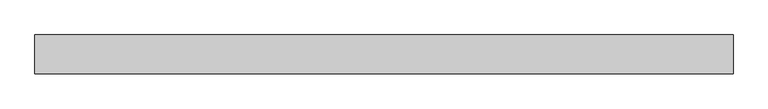
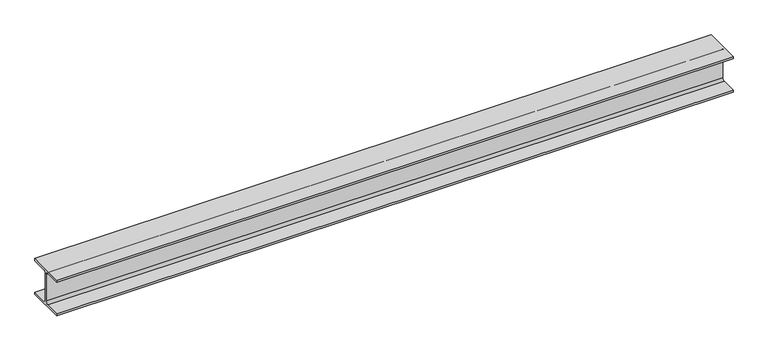
"""IFC4 building model written with IfcOpenShell, lengths in millimetres: beam geometry, 0912_Steel Framing_H-KSD3502 : H_SB_ASB_H-200x200x8x12."""

from ifc_helpers import new_model, si_unit, point, frame, frame_2d, origin, place, context, project, spatial, polyline, circle_curve, trimmed, segment, composite_curve, outline, extrude, source, transform, mapped, element, save


def beam_8ebba831(model_context):
    return source(origin(), model_context, "Body", "SweptSolid", [
        extrude(outline(composite_curve([segment(polyline([(100.0, -88.0), (100.0, -100.0), (-100.0, -100.0), (-100.0, -88.0), (-17.0, -88.0)]), True, "CONTINUOUS"), segment(trimmed(circle_curve(frame_2d((-17.0, -75.0)), 13.0), [point((-17.0, -88.0))], [point((-4.0, -75.0))], True, "CARTESIAN"), True, "CONTINUOUS"), segment(polyline([(-4.0, -75.0), (-4.0, 75.0)]), True, "CONTINUOUS"), segment(trimmed(circle_curve(frame_2d((-17.0, 75.0)), 13.0), [point((-4.0, 75.0))], [point((-17.0, 88.0))], True, "CARTESIAN"), True, "CONTINUOUS"), segment(polyline([(-17.0, 88.0), (-100.0, 88.0), (-100.0, 100.0), (100.0, 100.0), (100.0, 88.0), (17.0, 88.0)]), True, "CONTINUOUS"), segment(trimmed(circle_curve(frame_2d((17.0, 75.0)), 13.0), [point((17.0, 88.0))], [point((4.0, 75.0))], True, "CARTESIAN"), True, "CONTINUOUS"), segment(polyline([(4.0, 75.0), (4.0, -75.0)]), True, "CONTINUOUS"), segment(trimmed(circle_curve(frame_2d((17.0, -75.0)), 13.0), [point((4.0, -75.0))], [point((17.0, -88.0))], True, "CARTESIAN"), True, "CONTINUOUS"), segment(polyline([(17.0, -88.0), (100.0, -88.0)]), True, "CONTINUOUS")], self_intersect=False)), frame((-1849.7005928, 0.0, 0.0), z_axis=(1.0, 0.0, 0.0), x_axis=(0.0, 1.0, 0.0)), (0.0, 0.0, 1.0), 3573.4852126),
    ])


if __name__ == "__main__":
    model = new_model("IFC4")
    model_context = context("Model", 3, world=origin())
    ifc_project = project(units=[si_unit("LENGTHUNIT", "METRE", prefix="MILLI")], contexts=[model_context])
    site = spatial("IfcSite", under=ifc_project)
    building = spatial("IfcBuilding", under=site)
    placement = place(None, origin())
    beam_shape = beam_8ebba831(model_context)
    element("IfcBeam", 1, ObjectType="0912_Steel Framing_H-KSD3502 : H_SB_ASB_H-200x200x8x12", at=placement, inside=building, context=model_context, shape_type="MappedRepresentation", body=[
        mapped(beam_shape, transform((0.0, 0.0, 0.0), x_axis=(1.0, 0.0, 0.0), y_axis=(0.0, 1.0, 0.0), z_axis=(0.0, 0.0, 1.0))),
    ])
    save(model, "model.ifc")

# Revit data of these elements
# Type "0912_Steel Framing_H-KSD3502 : H_SB_ASB_H-200x200x8x12"
#   H_WM Code_1 = "S01AA002-00001 | Main Steel Structure Fabrication Work | Shelter/Building | Medium Steel - Standard (90KG/M>Weight≥30KG/M) | Material: (   )"
#   H_WM Code_2 = "S03AA028-00001 | Main Steel Structure Erection Work | Shelter/Building | Medium Steel (90KG/M>Weight≥30KG/M) | Material: (   )"
#   H_WM Code_3 = "S01AA010-00001 | Main Steel Structure Fabrication Work | Shelter/Building | Steel Painting/Coating | for Non-Fireproofed Steel Surface, Surface Preparation, Primer, Second & Final Coat | Material: (   )"
#   H_Q'ty Cal Type Tag = "SB-Q2"
#   Width = 20.0 cm
#   Web Thickness = 0.8 cm
#   Web Fillet = 1.3 cm
#   Warping Constant = 141000.0 cm⁶
#   W = 0
#   Torsional Moment of Inertia = 26.2485 cm⁴
#   Section Area = 63.53 cm²
#   Plastic Modulus weak axis = 244.0 cm³
#   Plastic Modulus strong axis = 525.0 cm³
#   Perimeter = 1.16 m²/m
#   Nominal Weight = 49.90 kgf/m
#   Moment of Inertia weak axis = 1600.00 cm⁴
#   Moment of Inertia strong axis = 4720.00 cm⁴
#   Height = 20.0 cm
#   Flange Thickness = 1.2 cm
#   Elastic Modulus weak axis = 160.0 cm³
#   Elastic Modulus strong axis = 472.0 cm³
#   Centroid Vertical = 10.0 cm
#   Centroid Horizontal = 10.0 cm
#   Ix = 47200000
#   Length [instance default] = 1.5240 m
#   Zx = 525000
#   b = 0.2000 m
#   h = 0.2000 m
#   r = 0.0130 m
#   s = 0.0080 m
#   t = 0.0120 m
#   A = 0.006353 m²
#   Structural Material [instance default] = Steel, 45-345
#   Assembly Code = ""
# Element 1 (IfcBeam, "0912_Steel Framing_H-KSD3502 : H_SB_ASB_H-200x200x8x12")
#   Structural Material = none
# Materials
#   "Steel, 45-345": class "Metal", colour RGB 189 187 185, transparency 0, Description = "Steel 345 MPa", Cost = 0
